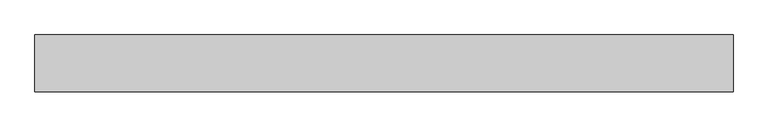
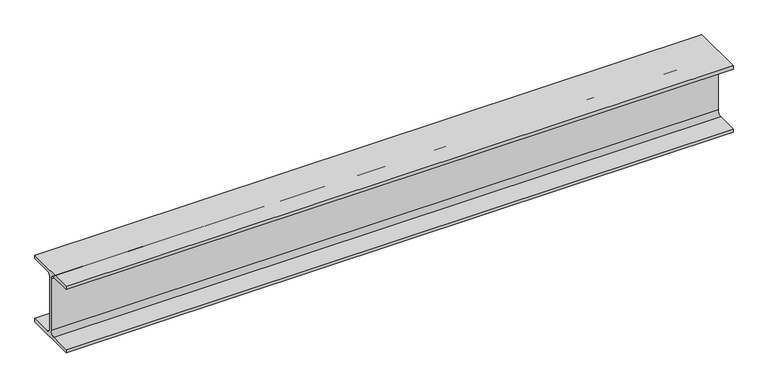
"""IFC4 building model written with IfcOpenShell, lengths in millimetres: beam geometry, 0912_Steel Framing_H-KSD3502 : H_SB_ASB_H-194x150x6x9."""

from ifc_helpers import new_model, si_unit, point, frame, frame_2d, origin, place, context, project, spatial, polyline, circle_curve, trimmed, segment, composite_curve, outline, extrude, source, transform, mapped, element, save


def beam_b633f717(model_context):
    return source(origin(), model_context, "Body", "SweptSolid", [
        extrude(outline(composite_curve([segment(polyline([(75.0, -88.0), (75.0, -97.0), (-75.0, -97.0), (-75.0, -88.0), (-16.0, -88.0)]), True, "CONTINUOUS"), segment(trimmed(circle_curve(frame_2d((-16.0, -75.0)), 13.0), [point((-16.0, -88.0))], [point((-3.0, -75.0))], True, "CARTESIAN"), True, "CONTINUOUS"), segment(polyline([(-3.0, -75.0), (-3.0, 75.0)]), True, "CONTINUOUS"), segment(trimmed(circle_curve(frame_2d((-16.0, 75.0)), 13.0), [point((-3.0, 75.0))], [point((-16.0, 88.0))], True, "CARTESIAN"), True, "CONTINUOUS"), segment(polyline([(-16.0, 88.0), (-75.0, 88.0), (-75.0, 97.0), (75.0, 97.0), (75.0, 88.0), (16.0, 88.0)]), True, "CONTINUOUS"), segment(trimmed(circle_curve(frame_2d((16.0, 75.0)), 13.0), [point((16.0, 88.0))], [point((3.0, 75.0))], True, "CARTESIAN"), True, "CONTINUOUS"), segment(polyline([(3.0, 75.0), (3.0, -75.0)]), True, "CONTINUOUS"), segment(trimmed(circle_curve(frame_2d((16.0, -75.0)), 13.0), [point((3.0, -75.0))], [point((16.0, -88.0))], True, "CARTESIAN"), True, "CONTINUOUS"), segment(polyline([(16.0, -88.0), (75.0, -88.0)]), True, "CONTINUOUS")], self_intersect=False)), frame((-853.4240734, 0.0, 0.0), z_axis=(1.0, 0.0, 0.0), x_axis=(0.0, 1.0, 0.0)), (0.0, 0.0, 1.0), 1846.5746098),
    ])


if __name__ == "__main__":
    model = new_model("IFC4")
    model_context = context("Model", 3, world=origin())
    ifc_project = project(units=[si_unit("LENGTHUNIT", "METRE", prefix="MILLI")], contexts=[model_context])
    site = spatial("IfcSite", under=ifc_project)
    building = spatial("IfcBuilding", under=site)
    placement = place(None, origin())
    beam_shape = beam_b633f717(model_context)
    element("IfcBeam", 1, ObjectType="0912_Steel Framing_H-KSD3502 : H_SB_ASB_H-194x150x6x9", at=placement, inside=building, context=model_context, shape_type="MappedRepresentation", body=[
        mapped(beam_shape, transform((0.0, 0.0, 0.0), x_axis=(1.0, 0.0, 0.0), y_axis=(0.0, 1.0, 0.0), z_axis=(0.0, 0.0, 1.0))),
    ])
    save(model, "model.ifc")

# Revit data of these elements
# Type "0912_Steel Framing_H-KSD3502 : H_SB_ASB_H-194x150x6x9"
#   H_WM Code_1 = "S01AA002-00001 | Main Steel Structure Fabrication Work | Shelter/Building | Medium Steel - Standard (90KG/M>Weight≥30KG/M) | Material: (   )"
#   H_WM Code_2 = "S03AA028-00001 | Main Steel Structure Erection Work | Shelter/Building | Medium Steel (90KG/M>Weight≥30KG/M) | Material: (   )"
#   H_WM Code_3 = "S01AA010-00001 | Main Steel Structure Fabrication Work | Shelter/Building | Steel Painting/Coating | for Non-Fireproofed Steel Surface, Surface Preparation, Primer, Second & Final Coat | Material: (   )"
#   H_Q'ty Cal Type Tag = "SB-Q2"
#   Width = 15.0 cm
#   Web Thickness = 0.6 cm
#   Web Fillet = 1.3 cm
#   Warping Constant = 43316.0 cm⁶
#   W = 0
#   Torsional Moment of Inertia = 8.622 cm⁴
#   Section Area = 39.01 cm²
#   Plastic Modulus weak axis = 104.0 cm³
#   Plastic Modulus strong axis = 309.0 cm³
#   Perimeter = 0.95 m²/m
#   Nominal Weight = 30.60 kgf/m
#   Moment of Inertia weak axis = 507.00 cm⁴
#   Moment of Inertia strong axis = 2690.00 cm⁴
#   Height = 19.4 cm
#   Flange Thickness = 0.9 cm
#   Elastic Modulus weak axis = 67.6 cm³
#   Elastic Modulus strong axis = 277.0 cm³
#   Centroid Vertical = 9.7 cm
#   Centroid Horizontal = 7.5 cm
#   Ix = 26900000
#   Length [instance default] = 1.5240 m
#   Zx = 309000
#   b = 0.1500 m
#   h = 0.1940 m
#   r = 0.0130 m
#   s = 0.0060 m
#   t = 0.0090 m
#   A = 0.003901 m²
#   Structural Material [instance default] = Steel, 45-345
#   Assembly Code = ""
# Element 1 (IfcBeam, "0912_Steel Framing_H-KSD3502 : H_SB_ASB_H-194x150x6x9")
#   Structural Material = none
# Materials
#   "Steel, 45-345": class "Metal", colour RGB 189 187 185, transparency 0, Description = "Steel 345 MPa", Cost = 0
